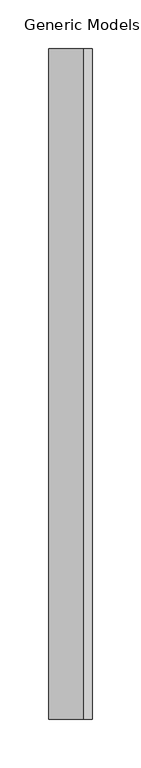
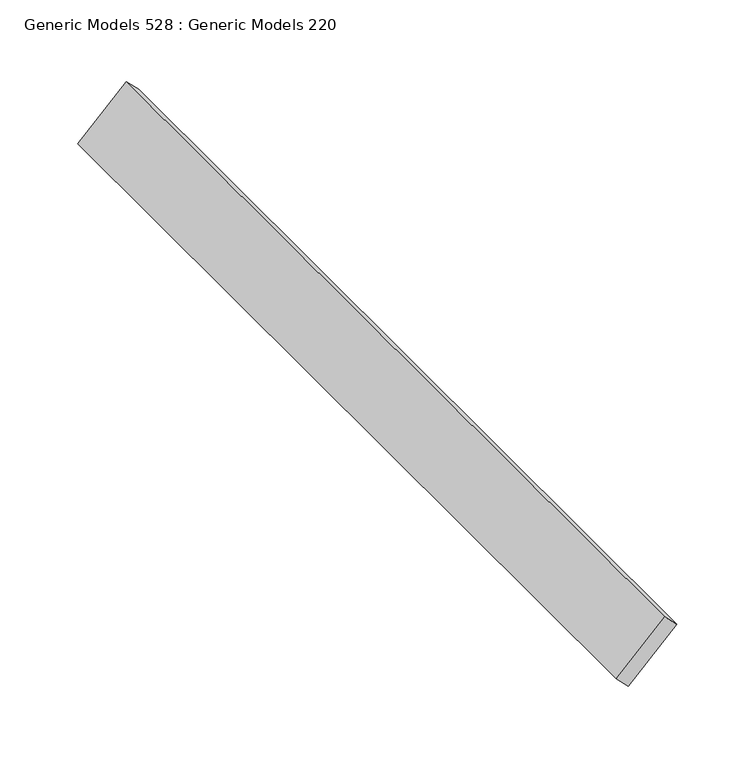
"""IFC4 building model written with IfcOpenShell, lengths in millimetres: proxy geometry, Generic Models 528 : Generic Models 220."""

from ifc_helpers import new_model, si_unit, frame, origin, place, context, project, spatial, polyline, outline, extrude, source, transform, mapped, element, save


def generic_models_528_generic_models_220_21915794(model_context):
    return source(origin(), model_context, "Body", "SweptSolid", [
        extrude(outline(polyline([(0.0, -12.7000001), (0.0, 0.0), (690.8142348, 0.0), (690.8142348, -12.7000001), (0.0, -12.7000001)])), frame((7841.3059863, 4539.4872686, 125382.6399101), z_axis=(0.7071067811868034, 0.0, 0.7071067811862918), x_axis=(0.0, -1.0, 0.0)), (0.0, 0.0, 1.0), 50.8),
    ])


if __name__ == "__main__":
    model = new_model("IFC4")
    model_context = context("Model", 3, world=origin())
    ifc_project = project(units=[si_unit("LENGTHUNIT", "METRE", prefix="MILLI")], contexts=[model_context])
    site = spatial("IfcSite", under=ifc_project)
    building = spatial("IfcBuilding", under=site)
    placement = place(None, origin())
    generic_models_528_generic_models_220_shape = generic_models_528_generic_models_220_21915794(model_context)
    element("IfcBuildingElementProxy", 1, Name="Generic Models 528 : Generic Models 220", ObjectType="Generic Models 528 : Generic Models 220", at=placement, inside=building, context=model_context, shape_type="MappedRepresentation", body=[
        mapped(generic_models_528_generic_models_220_shape, transform((0.0, 0.0, 0.0), x_axis=(1.0, 0.0, 0.0), y_axis=(0.0, 1.0, 0.0), z_axis=(0.0, 0.0, 1.0))),
    ])
    save(model, "model.ifc")

# Revit data of these elements
# Element 1 (IfcBuildingElementProxy, "Generic Models 528 : Generic Models 220")
#   Materials on its faces: "_WOOD TONE ALUMINUM EXTRUSION SLAT BY KNOTWOOD"
# Materials
#   "_WOOD TONE ALUMINUM EXTRUSION SLAT BY KNOTWOOD": class "Generic", colour RGB 177 130 114, transparency 0, Cost = 0
